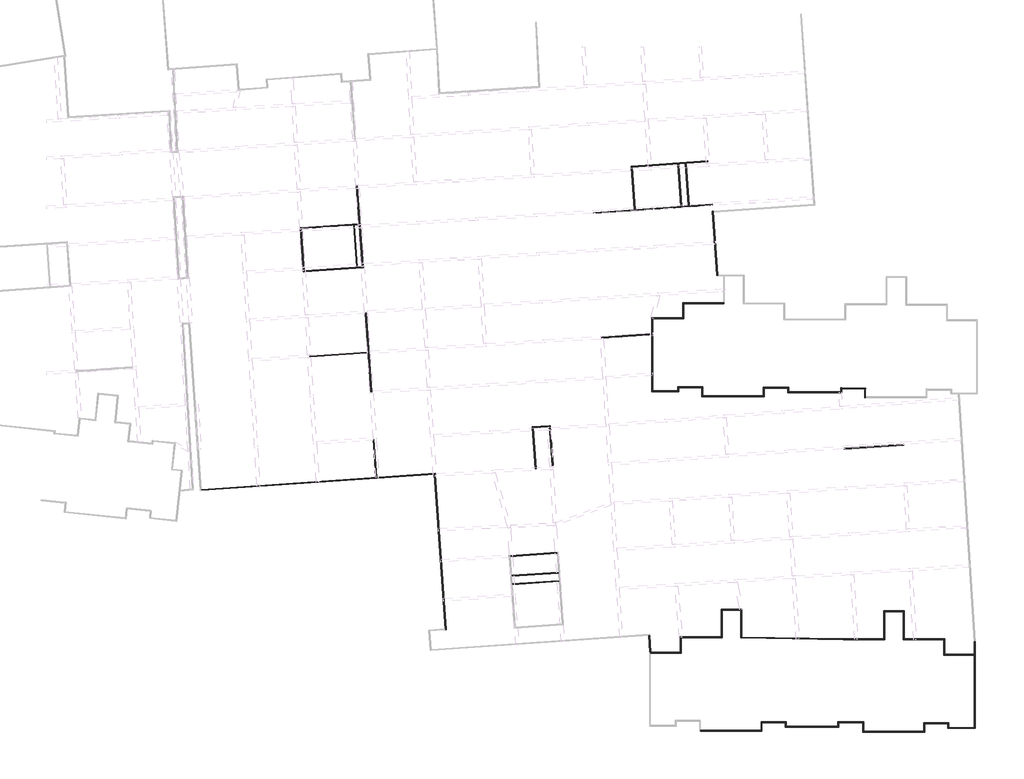
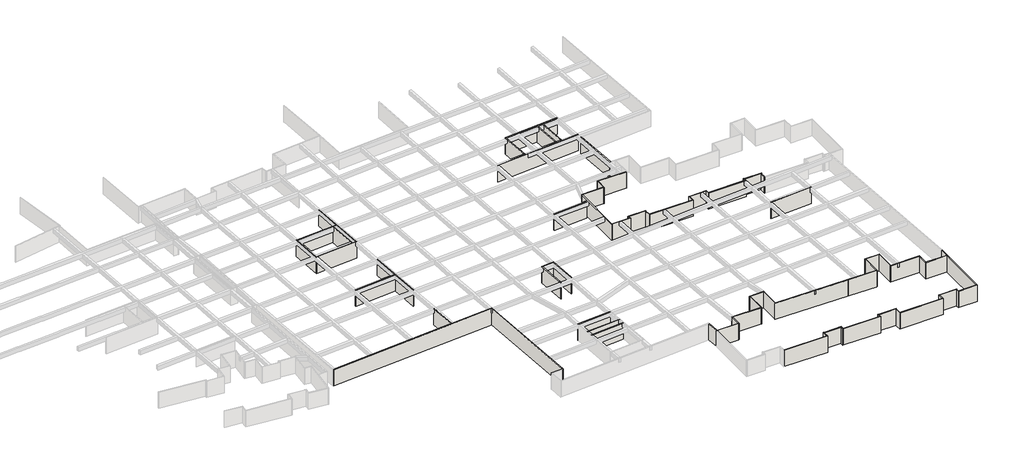
# One storey, part 5 of 14: 69 walls.
"""IFC4 building model written with IfcOpenShell, lengths in millimetres."""

from ifc_helpers import new_model, si_unit, origin, origin_with_axes, place, context, project, spatial, polyline, outline, extrude, faceted_brep, element, save

model = new_model("IFC4")

# Units and contexts
model_context = context("Model", 3, world=origin())
ifc_project = project(units=[si_unit("LENGTHUNIT", "METRE", prefix="MILLI")], contexts=[model_context])

# Site, building, storey
site = spatial("IfcSite", under=ifc_project)
building = spatial("IfcBuilding", under=site)
storey = spatial("IfcBuildingStorey", under=building, Name="户型图", Elevation=0.0)

# Walls
placement = place(None, origin())
element("IfcWall", 1, ObjectType="所有墙体", at=placement, inside=storey, context=model_context, shape_type="Brep", body=[
    faceted_brep([(-67010.794427, -211582.679776, 0.0), (-58619.9111457, -211582.679776, 0.0), (-58619.9111457, -211582.679776, 3300.0), (-67010.794427, -211582.679776, 3300.0), (-67010.794427, -211462.679776, 0.0), (-67010.794427, -211462.679776, 3300.0), (-58739.9111457, -211462.679776, 3300.0), (-58619.9111457, -211462.679776, 3300.0), (-58619.9111457, -211462.679776, 0.0), (-58739.9111457, -211462.679776, 0.0)], [[[0, 1, 2, 3]], [[4, 5, 6, 7, 8, 9]], [[1, 0, 4, 9, 8]], [[3, 2, 7, 6, 5]], [[0, 3, 5, 4]], [[2, 1, 8, 7]]]),
])
element("IfcWall", 2, ObjectType="所有墙体", at=placement, inside=storey, context=model_context, shape_type="Brep", body=[
    faceted_brep([(-58619.9111457, -211462.679776, 0.0), (-58619.9111457, -210441.7795098, 0.0), (-58619.9111457, -210321.7795098, 0.0), (-58619.9111457, -210321.7795098, 3300.0), (-58619.9111457, -210441.7795098, 3300.0), (-58619.9111457, -211462.679776, 3300.0), (-58739.9111457, -211462.679776, 0.0), (-58739.9111457, -211462.679776, 3300.0), (-58739.9111457, -210321.7795098, 3300.0), (-58739.9111457, -210321.7795098, 0.0)], [[[0, 1, 2, 3, 4, 5]], [[6, 7, 8, 9]], [[2, 1, 0, 6, 9]], [[5, 4, 3, 8, 7]], [[0, 5, 7, 6]], [[3, 2, 9, 8]]]),
])
element("IfcWall", 3, ObjectType="所有墙体", at=placement, inside=storey, context=model_context, shape_type="Brep", body=[
    faceted_brep([(-58619.9111457, -210441.7795098, 0.0), (-55431.7894255, -210441.7795098, 0.0), (-55311.7894255, -210441.7795098, 0.0), (-55311.7894255, -210441.7795098, 3300.0), (-55431.7894255, -210441.7795098, 3300.0), (-58619.9111457, -210441.7795098, 3300.0), (-58619.9111457, -210321.7795098, 0.0), (-58619.9111457, -210321.7795098, 3300.0), (-55311.7894255, -210321.7795098, 3300.0), (-55311.7894255, -210321.7795098, 0.0)], [[[0, 1, 2, 3, 4, 5]], [[6, 7, 8, 9]], [[2, 1, 0, 6, 9]], [[5, 4, 3, 8, 7]], [[0, 5, 7, 6]], [[3, 2, 9, 8]]]),
])
element("IfcWall", 4, ObjectType="所有墙体", at=placement, inside=storey, context=model_context, shape_type="Brep", body=[
    faceted_brep([(-55431.7894255, -210441.7795098, 0.0), (-55431.7894255, -211065.1063364, 0.0), (-55431.7894255, -211065.1063364, 3300.0), (-55431.7894255, -210441.7795098, 3300.0), (-55311.7894255, -210441.7795098, 0.0), (-55311.7894255, -210441.7795098, 3300.0), (-55311.7894255, -210945.1063364, 3300.0), (-55311.7894255, -211065.1063364, 3300.0), (-55311.7894255, -211065.1063364, 0.0), (-55311.7894255, -210945.1063364, 0.0)], [[[0, 1, 2, 3]], [[4, 5, 6, 7, 8, 9]], [[1, 0, 4, 9, 8]], [[3, 2, 7, 6, 5]], [[0, 3, 5, 4]], [[2, 1, 8, 7]]]),
])
element("IfcWall", 5, ObjectType="所有墙体", at=placement, inside=storey, context=model_context, shape_type="Brep", body=[
    faceted_brep([(-55311.7894255, -211065.1063364, 0.0), (-48116.0031651, -211065.1063364, 0.0), (-48116.0031651, -211065.1063364, 3300.0), (-55311.7894255, -211065.1063364, 3300.0), (-55311.7894255, -210945.1063364, 0.0), (-55311.7894255, -210945.1063364, 3300.0), (-48236.0031651, -210945.1063364, 3300.0), (-48116.0031651, -210945.1063364, 3300.0), (-48116.0031651, -210945.1063364, 0.0), (-48236.0031651, -210945.1063364, 0.0)], [[[0, 1, 2, 3]], [[4, 5, 6, 7, 8, 9]], [[1, 0, 4, 9, 8]], [[3, 2, 7, 6, 5]], [[0, 3, 5, 4]], [[2, 1, 8, 7]]]),
])
element("IfcWall", 6, ObjectType="所有墙体", at=placement, inside=storey, context=model_context, shape_type="Brep", body=[
    faceted_brep([(-48116.0031651, -210945.1063364, 0.0), (-48116.0031651, -210441.7795098, 0.0), (-48116.0031651, -210321.7795098, 0.0), (-48116.0031651, -210321.7795098, 3300.0), (-48116.0031651, -210441.7795098, 3300.0), (-48116.0031651, -210945.1063364, 3300.0), (-48236.0031651, -210945.1063364, 0.0), (-48236.0031651, -210945.1063364, 3300.0), (-48236.0031651, -210321.7795098, 3300.0), (-48236.0031651, -210321.7795098, 0.0)], [[[0, 1, 2, 3, 4, 5]], [[6, 7, 8, 9]], [[2, 1, 0, 6, 9]], [[5, 4, 3, 8, 7]], [[0, 5, 7, 6]], [[3, 2, 9, 8]]]),
])
element("IfcWall", 7, ObjectType="所有墙体", at=placement, inside=storey, context=model_context, shape_type="Brep", body=[
    faceted_brep([(-48116.0031651, -210441.7795098, 0.0), (-44836.0031651, -210441.7795098, 0.0), (-44716.0031651, -210441.7795098, 0.0), (-44716.0031651, -210441.7795098, 3300.0), (-44836.0031651, -210441.7795098, 3300.0), (-48116.0031651, -210441.7795098, 3300.0), (-48116.0031651, -210321.7795098, 0.0), (-48116.0031651, -210321.7795098, 3300.0), (-44716.0031651, -210321.7795098, 3300.0), (-44716.0031651, -210321.7795098, 0.0)], [[[0, 1, 2, 3, 4, 5]], [[6, 7, 8, 9]], [[2, 1, 0, 6, 9]], [[5, 4, 3, 8, 7]], [[0, 5, 7, 6]], [[3, 2, 9, 8]]]),
])
element("IfcWall", 8, ObjectType="所有墙体", at=placement, inside=storey, context=model_context, shape_type="Brep", body=[
    faceted_brep([(-44836.0031651, -210441.7795098, 0.0), (-44836.0031651, -211739.788444, 0.0), (-44836.0031651, -211739.788444, 3300.0), (-44836.0031651, -210441.7795098, 3300.0), (-44716.0031651, -210441.7795098, 0.0), (-44716.0031651, -210441.7795098, 3300.0), (-44716.0031651, -211619.788444, 3300.0), (-44716.0031651, -211739.788444, 3300.0), (-44716.0031651, -211739.788444, 0.0), (-44716.0031651, -211619.788444, 0.0)], [[[0, 1, 2, 3]], [[4, 5, 6, 7, 8, 9]], [[1, 0, 4, 9, 8]], [[3, 2, 7, 6, 5]], [[0, 3, 5, 4]], [[2, 1, 8, 7]]]),
])
element("IfcWall", 9, ObjectType="所有墙体", at=placement, inside=storey, context=model_context, shape_type="Brep", body=[
    faceted_brep([(-44716.0031651, -211739.788444, 0.0), (-36420.4670689, -211739.788444, 0.0), (-36420.4670689, -211739.788444, 3300.0), (-44716.0031651, -211739.788444, 3300.0), (-44716.0031651, -211619.788444, 0.0), (-44716.0031651, -211619.788444, 3300.0), (-36540.4670689, -211619.788444, 3300.0), (-36420.4670689, -211619.788444, 3300.0), (-36420.4670689, -211619.788444, 0.0), (-36540.4670689, -211619.788444, 0.0)], [[[0, 1, 2, 3]], [[4, 5, 6, 7, 8, 9]], [[1, 0, 4, 9, 8]], [[3, 2, 7, 6, 5]], [[0, 3, 5, 4]], [[2, 1, 8, 7]]]),
])
element("IfcWall", 10, ObjectType="所有墙体", at=placement, inside=storey, context=model_context, shape_type="Brep", body=[
    faceted_brep([(-36420.4670689, -211619.788444, 0.0), (-36420.4670689, -210598.2162779, 0.0), (-36420.4670689, -210478.2162779, 0.0), (-36420.4670689, -210478.2162779, 3300.0), (-36420.4670689, -210598.2162779, 3300.0), (-36420.4670689, -211619.788444, 3300.0), (-36540.4670689, -211619.788444, 0.0), (-36540.4670689, -211619.788444, 3300.0), (-36540.4670689, -210478.2162779, 3300.0), (-36540.4670689, -210478.2162779, 0.0)], [[[0, 1, 2, 3, 4, 5]], [[6, 7, 8, 9]], [[2, 1, 0, 6, 9]], [[5, 4, 3, 8, 7]], [[0, 5, 7, 6]], [[3, 2, 9, 8]]]),
])
element("IfcWall", 11, ObjectType="所有墙体", at=placement, inside=storey, context=model_context, shape_type="Brep", body=[
    faceted_brep([(-36420.4670689, -210598.2162779, 0.0), (-33232.340614, -210598.2162779, 0.0), (-33112.340614, -210598.2162779, 0.0), (-33112.340614, -210598.2162779, 3300.0), (-33232.340614, -210598.2162779, 3300.0), (-36420.4670689, -210598.2162779, 3300.0), (-36420.4670689, -210478.2162779, 0.0), (-36420.4670689, -210478.2162779, 3300.0), (-33112.340614, -210478.2162779, 3300.0), (-33112.340614, -210478.2162779, 0.0)], [[[0, 1, 2, 3, 4, 5]], [[6, 7, 8, 9]], [[2, 1, 0, 6, 9]], [[5, 4, 3, 8, 7]], [[0, 5, 7, 6]], [[3, 2, 9, 8]]]),
])
element("IfcWall", 12, ObjectType="所有墙体", at=placement, inside=storey, context=model_context, shape_type="Brep", body=[
    faceted_brep([(-33232.340614, -210598.2162779, 0.0), (-33232.340614, -211221.5431378, 0.0), (-33232.340614, -211221.5431378, 3300.0), (-33232.340614, -210598.2162779, 3300.0), (-33112.340614, -210598.2162779, 0.0), (-33112.340614, -210598.2162779, 3300.0), (-33112.340614, -211101.5431378, 3300.0), (-33112.340614, -211221.5431378, 3300.0), (-33112.340614, -211221.5431378, 0.0), (-33112.340614, -211101.5431378, 0.0)], [[[0, 1, 2, 3]], [[4, 5, 6, 7, 8, 9]], [[1, 0, 4, 9, 8]], [[3, 2, 7, 6, 5]], [[0, 3, 5, 4]], [[2, 1, 8, 7]]]),
])
element("IfcWall", 13, ObjectType="所有墙体", at=placement, inside=storey, context=model_context, shape_type="Brep", body=[
    faceted_brep([(-33112.340614, -211221.5431378, 0.0), (-29516.643738, -211221.5431378, 0.0), (-29516.643738, -211221.5431378, 3300.0), (-33112.340614, -211221.5431378, 3300.0), (-33112.340614, -211101.5431378, 0.0), (-33112.340614, -211101.5431378, 3300.0), (-29636.643738, -211101.5431378, 3300.0), (-29516.643738, -211101.5431378, 3300.0), (-29516.643738, -211101.5431378, 0.0), (-29636.643738, -211101.5431378, 0.0)], [[[0, 1, 2, 3]], [[4, 5, 6, 7, 8, 9]], [[1, 0, 4, 9, 8]], [[3, 2, 7, 6, 5]], [[0, 3, 5, 4]], [[2, 1, 8, 7]]]),
])
element("IfcWall", 14, ObjectType="所有墙体", at=placement, inside=storey, context=model_context, shape_type="Brep", body=[
    faceted_brep([(-29516.643738, -211101.5431378, 0.0), (-29516.643738, -199359.5961168, 0.0), (-29516.643738, -199359.5961168, 3300.0), (-29516.643738, -211101.5431378, 3300.0), (-29636.643738, -211101.5431378, 0.0), (-29636.643738, -211101.5431378, 3300.0), (-29636.643738, -201221.5431378, 3300.0), (-29636.643738, -201101.5431378, 3300.0), (-29636.643738, -199363.4901589, 3300.0), (-29636.643738, -199363.4901589, 0.0), (-29636.643738, -201101.5431378, 0.0), (-29636.643738, -201221.5431378, 0.0)], [[[0, 1, 2, 3]], [[4, 5, 6, 7, 8, 9, 10, 11]], [[1, 0, 4, 11, 10, 9]], [[3, 2, 8, 7, 6, 5]], [[0, 3, 5, 4]], [[2, 1, 9, 8]]]),
])
element("IfcWall", 15, ObjectType="所有墙体", at=placement, inside=storey, context=model_context, shape_type="Brep", body=[
    faceted_brep([(-29636.643738, -201101.5431378, 0.0), (-33646.2792422, -201101.5431378, 0.0), (-33766.2792422, -201101.5431378, 0.0), (-33766.2792422, -201101.5431378, 3300.0), (-33646.2792422, -201101.5431378, 3300.0), (-29636.643738, -201101.5431378, 3300.0), (-29636.643738, -201221.5431378, 0.0), (-29636.643738, -201221.5431378, 3300.0), (-33766.2792422, -201221.5431378, 3300.0), (-33766.2792422, -201221.5431378, 0.0)], [[[0, 1, 2, 3, 4, 5]], [[6, 7, 8, 9]], [[2, 1, 0, 6, 9]], [[5, 4, 3, 8, 7]], [[0, 5, 7, 6]], [[3, 2, 9, 8]]]),
])
element("IfcWall", 16, ObjectType="所有墙体", at=placement, inside=storey, context=model_context, shape_type="Brep", body=[
    faceted_brep([(-33646.2792422, -201101.5431378, 0.0), (-33646.2792422, -198997.4801078, 0.0), (-33646.2792422, -198997.4801078, 3300.0), (-33646.2792422, -201101.5431378, 3300.0), (-33766.2792422, -201101.5431378, 0.0), (-33766.2792422, -201101.5431378, 3300.0), (-33766.2792422, -199117.4801078, 3300.0), (-33766.2792422, -198997.4801078, 3300.0), (-33766.2792422, -198997.4801078, 0.0), (-33766.2792422, -199117.4801078, 0.0)], [[[0, 1, 2, 3]], [[4, 5, 6, 7, 8, 9]], [[1, 0, 4, 9, 8]], [[3, 2, 7, 6, 5]], [[0, 3, 5, 4]], [[2, 1, 8, 7]]]),
])
element("IfcWall", 17, ObjectType="所有墙体", at=placement, inside=storey, context=model_context, shape_type="Brep", body=[
    faceted_brep([(-33766.2792422, -198997.4801078, 0.0), (-39181.5899679, -198997.4801078, 0.0), (-39301.5899679, -198997.4801078, 0.0), (-39301.5899679, -198997.4801078, 3300.0), (-39181.5899679, -198997.4801078, 3300.0), (-33766.2792422, -198997.4801078, 3300.0), (-33766.2792422, -199117.4801078, 0.0), (-33766.2792422, -199117.4801078, 3300.0), (-39301.5899679, -199117.4801078, 3300.0), (-39301.5899679, -199117.4801078, 0.0)], [[[0, 1, 2, 3, 4, 5]], [[6, 7, 8, 9]], [[2, 1, 0, 6, 9]], [[5, 4, 3, 8, 7]], [[0, 5, 7, 6]], [[3, 2, 9, 8]]]),
])
element("IfcWall", 18, ObjectType="所有墙体", at=placement, inside=storey, context=model_context, shape_type="Brep", body=[
    faceted_brep([(-39181.5899679, -198997.4801078, 0.0), (-39181.5899679, -195158.3790997, 0.0), (-39181.5899679, -195158.3790997, 3300.0), (-39181.5899679, -198997.4801078, 3300.0), (-39301.5899679, -198997.4801078, 0.0), (-39301.5899679, -198997.4801078, 3300.0), (-39301.5899679, -195278.3790997, 3300.0), (-39301.5899679, -195158.3790997, 3300.0), (-39301.5899679, -195158.3790997, 0.0), (-39301.5899679, -195278.3790997, 0.0)], [[[0, 1, 2, 3]], [[4, 5, 6, 7, 8, 9]], [[1, 0, 4, 9, 8]], [[3, 2, 7, 6, 5]], [[0, 3, 5, 4]], [[2, 1, 8, 7]]]),
])
element("IfcWall", 19, ObjectType="所有墙体", at=placement, inside=storey, context=model_context, shape_type="Brep", body=[
    faceted_brep([(-39301.5899679, -195158.3790997, 0.0), (-41974.6033306, -195158.3790997, 0.0), (-41974.6033306, -195158.3790997, 3300.0), (-39301.5899679, -195158.3790997, 3300.0), (-39301.5899679, -195278.3790997, 0.0), (-39301.5899679, -195278.3790997, 3300.0), (-41854.6033306, -195278.3790997, 3300.0), (-41974.6033306, -195278.3790997, 3300.0), (-41974.6033306, -195278.3790997, 0.0), (-41854.6033306, -195278.3790997, 0.0)], [[[0, 1, 2, 3]], [[4, 5, 6, 7, 8, 9]], [[1, 0, 4, 9, 8]], [[3, 2, 7, 6, 5]], [[0, 3, 5, 4]], [[2, 1, 8, 7]]]),
])
element("IfcWall", 20, ObjectType="所有墙体", at=placement, inside=storey, context=model_context, shape_type="Brep", body=[
    faceted_brep([(-41974.6033306, -195278.3790997, 0.0), (-41974.6033306, -198997.4801078, 0.0), (-41974.6033306, -199117.4801078, 0.0), (-41974.6033306, -199117.4801078, 3300.0), (-41974.6033306, -198997.4801078, 3300.0), (-41974.6033306, -195278.3790997, 3300.0), (-41854.6033306, -195278.3790997, 0.0), (-41854.6033306, -195278.3790997, 3300.0), (-41854.6033306, -199117.4801078, 3300.0), (-41854.6033306, -199117.4801078, 0.0)], [[[0, 1, 2, 3, 4, 5]], [[6, 7, 8, 9]], [[2, 1, 0, 6, 9]], [[5, 4, 3, 8, 7]], [[0, 5, 7, 6]], [[3, 2, 9, 8]]]),
])
element("IfcWall", 21, ObjectType="所有墙体", at=placement, inside=storey, context=model_context, shape_type="SweptSolid", body=[
    extrude(outline(polyline([(-47491.2711945, -198997.4801078), (-41974.6033306, -198997.4801078), (-41974.6033306, -199117.4801078), (-47492.3184187, -199117.4801078), (-47491.2711945, -198997.4801078)])), origin_with_axes(), (0.0, 0.0, 1.0), 3300.0),
])
element("IfcWall", 22, ObjectType="所有墙体", at=placement, inside=storey, context=model_context, shape_type="Brep", body=[
    faceted_brep([(-47491.2711945, -198997.4801078, 0.0), (-61380.425437, -198755.0440187, 0.0), (-61500.425437, -198752.9494109, 0.0), (-61500.425437, -198752.9494109, 3300.0), (-61380.425437, -198755.0440187, 3300.0), (-47491.2711945, -198997.4801078, 3300.0), (-47492.3184187, -199117.4801078, 0.0), (-47492.3184187, -199117.4801078, 3300.0), (-61500.425437, -198872.9676903, 3300.0), (-61500.425437, -198872.9676903, 0.0)], [[[0, 1, 2, 3, 4, 5]], [[6, 7, 8, 9]], [[2, 1, 0, 6, 9]], [[5, 4, 3, 8, 7]], [[0, 5, 7, 6]], [[3, 2, 9, 8]]]),
])
element("IfcWall", 23, ObjectType="所有墙体", at=placement, inside=storey, context=model_context, shape_type="Brep", body=[
    faceted_brep([(-61380.425437, -198755.0440187, 0.0), (-61380.425437, -194954.0058545, 0.0), (-61380.425437, -194954.0058545, 3300.0), (-61380.425437, -198755.0440187, 3300.0), (-61500.425437, -198752.9494109, 0.0), (-61500.425437, -198752.9494109, 3300.0), (-61500.425437, -195074.0058545, 3300.0), (-61500.425437, -194954.0058545, 3300.0), (-61500.425437, -194954.0058545, 0.0), (-61500.425437, -195074.0058545, 0.0)], [[[0, 1, 2, 3]], [[4, 5, 6, 7, 8, 9]], [[1, 0, 4, 9, 8]], [[3, 2, 7, 6, 5]], [[0, 3, 5, 4]], [[2, 1, 8, 7]]]),
])
element("IfcWall", 24, ObjectType="所有墙体", at=placement, inside=storey, context=model_context, shape_type="Brep", body=[
    faceted_brep([(-61500.425437, -194954.0058545, 0.0), (-64173.7143397, -194954.0058545, 0.0), (-64173.7143397, -194954.0058545, 3300.0), (-61500.425437, -194954.0058545, 3300.0), (-61500.425437, -195074.0058545, 0.0), (-61500.425437, -195074.0058545, 3300.0), (-64053.7143397, -195074.0058545, 3300.0), (-64173.7143397, -195074.0058545, 3300.0), (-64173.7143397, -195074.0058545, 0.0), (-64053.7143397, -195074.0058545, 0.0)], [[[0, 1, 2, 3]], [[4, 5, 6, 7, 8, 9]], [[1, 0, 4, 9, 8]], [[3, 2, 7, 6, 5]], [[0, 3, 5, 4]], [[2, 1, 8, 7]]]),
])
element("IfcWall", 25, ObjectType="所有墙体", at=placement, inside=storey, context=model_context, shape_type="Brep", body=[
    faceted_brep([(-64173.7143397, -195074.0058545, 0.0), (-64173.7143397, -198707.3434231, 0.0), (-64173.7143397, -198827.3434231, 0.0), (-64173.7143397, -198827.3434231, 3300.0), (-64173.7143397, -198707.3434231, 3300.0), (-64173.7143397, -195074.0058545, 3300.0), (-64053.7143397, -195074.0058545, 0.0), (-64053.7143397, -195074.0058545, 3300.0), (-64053.7143397, -198827.3434231, 3300.0), (-64053.7143397, -198827.3434231, 0.0)], [[[0, 1, 2, 3, 4, 5]], [[6, 7, 8, 9]], [[2, 1, 0, 6, 9]], [[5, 4, 3, 8, 7]], [[0, 5, 7, 6]], [[3, 2, 9, 8]]]),
])
element("IfcWall", 26, ObjectType="所有墙体", at=placement, inside=storey, context=model_context, shape_type="Brep", body=[
    faceted_brep([(-64173.7143397, -198707.3434231, 0.0), (-69750.3014513, -198707.3434231, 0.0), (-69750.3014513, -198707.3434231, 3300.0), (-64173.7143397, -198707.3434231, 3300.0), (-64173.7143397, -198827.3434231, 0.0), (-64173.7143397, -198827.3434231, 3300.0), (-69630.3014513, -198827.3434231, 3300.0), (-69750.3014513, -198827.3434231, 3300.0), (-69750.3014513, -198827.3434231, 0.0), (-69630.3014513, -198827.3434231, 0.0)], [[[0, 1, 2, 3]], [[4, 5, 6, 7, 8, 9]], [[1, 0, 4, 9, 8]], [[3, 2, 7, 6, 5]], [[0, 3, 5, 4]], [[2, 1, 8, 7]]]),
])
element("IfcWall", 27, ObjectType="所有墙体", at=placement, inside=storey, context=model_context, shape_type="Brep", body=[
    faceted_brep([(-69750.3014513, -198827.3434231, 0.0), (-69750.3014513, -200843.9572436, 0.0), (-69750.3014513, -200963.9572436, 0.0), (-69750.3014513, -200963.9572436, 3300.0), (-69750.3014513, -200843.9572436, 3300.0), (-69750.3014513, -198827.3434231, 3300.0), (-69630.3014513, -198827.3434231, 0.0), (-69630.3014513, -198827.3434231, 3300.0), (-69630.3014513, -200963.9572436, 3300.0), (-69630.3014513, -200963.9572436, 0.0)], [[[0, 1, 2, 3, 4, 5]], [[6, 7, 8, 9]], [[2, 1, 0, 6, 9]], [[5, 4, 3, 8, 7]], [[0, 5, 7, 6]], [[3, 2, 9, 8]]]),
])
element("IfcWall", 28, ObjectType="所有墙体", at=placement, inside=storey, context=model_context, shape_type="Brep", body=[
    faceted_brep([(-69750.3014513, -200843.9572436, 0.0), (-73794.4999662, -200843.9572436, 0.0), (-73845.252881, -200843.9572436, 0.0), (-73845.252881, -200843.9572436, 3300.0), (-73794.4999662, -200843.9572436, 3300.0), (-69750.3014513, -200843.9572436, 3300.0), (-69750.3014513, -200963.9572436, 0.0), (-69750.3014513, -200963.9572436, 3300.0), (-73845.252881, -200963.9572436, 3300.0), (-73845.252881, -200963.9572436, 0.0)], [[[0, 1, 2, 3, 4, 5]], [[6, 7, 8, 9]], [[2, 1, 0, 6, 9]], [[5, 4, 3, 8, 7]], [[3, 2, 9, 8]], [[0, 5, 7, 6]]]),
])
element("IfcWall", 29, ObjectType="所有墙体", at=placement, inside=storey, context=model_context, shape_type="Brep", body=[
    faceted_brep([(-63852.357784, -153118.7611434, 0.0), (-69429.0689186, -153118.7611434, 0.0), (-69429.0689186, -153118.7611434, 3300.0), (-63852.357784, -153118.7611434, 3300.0), (-63852.357784, -153238.7611434, 0.0), (-63852.357784, -153238.7611434, 3300.0), (-69309.0689186, -153238.7611434, 3300.0), (-69429.0689186, -153238.7611434, 3300.0), (-69429.0689186, -153238.7611434, 0.0), (-69309.0689186, -153238.7611434, 0.0)], [[[0, 1, 2, 3]], [[4, 5, 6, 7, 8, 9]], [[1, 0, 4, 9, 8]], [[3, 2, 7, 6, 5]], [[0, 3, 5, 4]], [[2, 1, 8, 7]]]),
])
element("IfcWall", 30, ObjectType="所有墙体", at=placement, inside=storey, context=model_context, shape_type="Brep", body=[
    faceted_brep([(-69429.0689186, -153238.7611434, 0.0), (-69429.0689186, -155179.8125449, 0.0), (-69429.0689186, -155299.8125449, 0.0), (-69429.0689186, -155299.8125449, 3300.0), (-69429.0689186, -155179.8125449, 3300.0), (-69429.0689186, -153238.7611434, 3300.0), (-69309.0689186, -153238.7611434, 0.0), (-69309.0689186, -153238.7611434, 3300.0), (-69309.0689186, -155299.8125449, 3300.0), (-69309.0689186, -155299.8125449, 0.0)], [[[0, 1, 2, 3, 4, 5]], [[6, 7, 8, 9]], [[2, 1, 0, 6, 9]], [[5, 4, 3, 8, 7]], [[0, 5, 7, 6]], [[3, 2, 9, 8]]]),
])
element("IfcWall", 31, ObjectType="所有墙体", at=placement, inside=storey, context=model_context, shape_type="Brep", body=[
    faceted_brep([(-69429.0689186, -155179.8125449, 0.0), (-73643.5852972, -155179.8125449, 0.0), (-73643.5852972, -155179.8125449, 3300.0), (-69429.0689186, -155179.8125449, 3300.0), (-69429.0689186, -155299.8125449, 0.0), (-69429.0689186, -155299.8125449, 3300.0), (-73523.5852972, -155299.8125449, 3300.0), (-73643.5852972, -155299.8125449, 3300.0), (-73643.5852972, -155299.8125449, 0.0), (-73523.5852972, -155299.8125449, 0.0)], [[[0, 1, 2, 3]], [[4, 5, 6, 7, 8, 9]], [[1, 0, 4, 9, 8]], [[3, 2, 7, 6, 5]], [[0, 3, 5, 4]], [[2, 1, 8, 7]]]),
])
element("IfcWall", 32, ObjectType="所有墙体", at=placement, inside=storey, context=model_context, shape_type="Brep", body=[
    faceted_brep([(-73643.5852972, -155299.8125449, 0.0), (-73643.5852972, -165270.5834458, 0.0), (-73643.5852972, -165270.5834458, 3300.0), (-73643.5852972, -155299.8125449, 3300.0), (-73523.5852972, -155299.8125449, 0.0), (-73523.5852972, -155299.8125449, 3300.0), (-73523.5852972, -165150.5834458, 3300.0), (-73523.5852972, -165270.5834458, 3300.0), (-73523.5852972, -165270.5834458, 0.0), (-73523.5852972, -165150.5834458, 0.0)], [[[0, 1, 2, 3]], [[4, 5, 6, 7, 8, 9]], [[1, 0, 4, 9, 8]], [[3, 2, 7, 6, 5]], [[0, 3, 5, 4]], [[2, 1, 8, 7]]]),
])
element("IfcWall", 33, ObjectType="所有墙体", at=placement, inside=storey, context=model_context, shape_type="Brep", body=[
    faceted_brep([(-73523.5852972, -165270.5834458, 0.0), (-69993.2264591, -165270.5834458, 0.0), (-69993.2264591, -165270.5834458, 3300.0), (-73523.5852972, -165270.5834458, 3300.0), (-73523.5852972, -165150.5834458, 0.0), (-73523.5852972, -165150.5834458, 3300.0), (-70113.2264591, -165150.5834458, 3300.0), (-69993.2264591, -165150.5834458, 3300.0), (-69993.2264591, -165150.5834458, 0.0), (-70113.2264591, -165150.5834458, 0.0)], [[[0, 1, 2, 3]], [[4, 5, 6, 7, 8, 9]], [[1, 0, 4, 9, 8]], [[3, 2, 7, 6, 5]], [[0, 3, 5, 4]], [[2, 1, 8, 7]]]),
])
element("IfcWall", 34, ObjectType="所有墙体", at=placement, inside=storey, context=model_context, shape_type="Brep", body=[
    faceted_brep([(-69993.2264591, -165150.5834458, 0.0), (-69993.2264591, -164695.2578452, 0.0), (-69993.2264591, -164575.2578452, 0.0), (-69993.2264591, -164575.2578452, 3300.0), (-69993.2264591, -164695.2578452, 3300.0), (-69993.2264591, -165150.5834458, 3300.0), (-70113.2264591, -165150.5834458, 0.0), (-70113.2264591, -165150.5834458, 3300.0), (-70113.2264591, -164575.2578452, 3300.0), (-70113.2264591, -164575.2578452, 0.0)], [[[0, 1, 2, 3, 4, 5]], [[6, 7, 8, 9]], [[2, 1, 0, 6, 9]], [[5, 4, 3, 8, 7]], [[0, 5, 7, 6]], [[3, 2, 9, 8]]]),
])
element("IfcWall", 35, ObjectType="所有墙体", at=placement, inside=storey, context=model_context, shape_type="Brep", body=[
    faceted_brep([(-69993.2264591, -164695.2578452, 0.0), (-66809.1223042, -164695.2578452, 0.0), (-66689.1223042, -164695.2578452, 0.0), (-66689.1223042, -164695.2578452, 3300.0), (-66809.1223042, -164695.2578452, 3300.0), (-69993.2264591, -164695.2578452, 3300.0), (-69993.2264591, -164575.2578452, 0.0), (-69993.2264591, -164575.2578452, 3300.0), (-66689.1223042, -164575.2578452, 3300.0), (-66689.1223042, -164575.2578452, 0.0)], [[[0, 1, 2, 3, 4, 5]], [[6, 7, 8, 9]], [[2, 1, 0, 6, 9]], [[5, 4, 3, 8, 7]], [[0, 5, 7, 6]], [[3, 2, 9, 8]]]),
])
element("IfcWall", 36, ObjectType="所有墙体", at=placement, inside=storey, context=model_context, shape_type="Brep", body=[
    faceted_brep([(-66809.1223042, -164695.2578452, 0.0), (-66809.1223042, -165918.39398, 0.0), (-66809.1223042, -165918.39398, 3300.0), (-66809.1223042, -164695.2578452, 3300.0), (-66689.1223042, -164695.2578452, 0.0), (-66689.1223042, -164695.2578452, 3300.0), (-66689.1223042, -165798.39398, 3300.0), (-66689.1223042, -165918.39398, 3300.0), (-66689.1223042, -165918.39398, 0.0), (-66689.1223042, -165798.39398, 0.0)], [[[0, 1, 2, 3]], [[4, 5, 6, 7, 8, 9]], [[1, 0, 4, 9, 8]], [[3, 2, 7, 6, 5]], [[0, 3, 5, 4]], [[2, 1, 8, 7]]]),
])
element("IfcWall", 37, ObjectType="所有墙体", at=placement, inside=storey, context=model_context, shape_type="Brep", body=[
    faceted_brep([(-66689.1223042, -165918.39398, 0.0), (-58297.4707286, -165918.39398, 0.0), (-58297.4707286, -165918.39398, 3300.0), (-66689.1223042, -165918.39398, 3300.0), (-66689.1223042, -165798.39398, 0.0), (-66689.1223042, -165798.39398, 3300.0), (-58417.4707286, -165798.39398, 3300.0), (-58297.4707286, -165798.39398, 3300.0), (-58297.4707286, -165798.39398, 0.0), (-58417.4707286, -165798.39398, 0.0)], [[[0, 1, 2, 3]], [[4, 5, 6, 7, 8, 9]], [[1, 0, 4, 9, 8]], [[3, 2, 7, 6, 5]], [[0, 3, 5, 4]], [[2, 1, 8, 7]]]),
])
element("IfcWall", 38, ObjectType="所有墙体", at=placement, inside=storey, context=model_context, shape_type="Brep", body=[
    faceted_brep([(-58297.4707286, -165798.39398, 0.0), (-58297.4707286, -164777.0504792, 0.0), (-58297.4707286, -164657.0504792, 0.0), (-58297.4707286, -164657.0504792, 3300.0), (-58297.4707286, -164777.0504792, 3300.0), (-58297.4707286, -165798.39398, 3300.0), (-58417.4707286, -165798.39398, 0.0), (-58417.4707286, -165798.39398, 3300.0), (-58417.4707286, -164657.0504792, 3300.0), (-58417.4707286, -164657.0504792, 0.0)], [[[0, 1, 2, 3, 4, 5]], [[6, 7, 8, 9]], [[2, 1, 0, 6, 9]], [[5, 4, 3, 8, 7]], [[0, 5, 7, 6]], [[3, 2, 9, 8]]]),
])
element("IfcWall", 39, ObjectType="所有墙体", at=placement, inside=storey, context=model_context, shape_type="Brep", body=[
    faceted_brep([(-58297.4707286, -164777.0504792, 0.0), (-55109.4082066, -164777.0504792, 0.0), (-54989.4082066, -164777.0504792, 0.0), (-54989.4082066, -164777.0504792, 3300.0), (-55109.4082066, -164777.0504792, 3300.0), (-58297.4707286, -164777.0504792, 3300.0), (-58297.4707286, -164657.0504792, 0.0), (-58297.4707286, -164657.0504792, 3300.0), (-54989.4082066, -164657.0504792, 3300.0), (-54989.4082066, -164657.0504792, 0.0)], [[[0, 1, 2, 3, 4, 5]], [[6, 7, 8, 9]], [[2, 1, 0, 6, 9]], [[5, 4, 3, 8, 7]], [[0, 5, 7, 6]], [[3, 2, 9, 8]]]),
])
element("IfcWall", 40, ObjectType="所有墙体", at=placement, inside=storey, context=model_context, shape_type="Brep", body=[
    faceted_brep([(-55109.4082066, -164777.0504792, 0.0), (-55109.4082066, -165400.1996242, 0.0), (-55109.4082066, -165400.1996242, 3300.0), (-55109.4082066, -164777.0504792, 3300.0), (-54989.4082066, -164777.0504792, 0.0), (-54989.4082066, -164777.0504792, 3300.0), (-54989.4082066, -165280.1996242, 3300.0), (-54989.4082066, -165400.1996242, 3300.0), (-54989.4082066, -165400.1996242, 0.0), (-54989.4082066, -165280.1996242, 0.0)], [[[0, 1, 2, 3]], [[4, 5, 6, 7, 8, 9]], [[1, 0, 4, 9, 8]], [[3, 2, 7, 6, 5]], [[0, 3, 5, 4]], [[2, 1, 8, 7]]]),
])
element("IfcWall", 41, ObjectType="所有墙体", at=placement, inside=storey, context=model_context, shape_type="Brep", body=[
    faceted_brep([(-54989.4082066, -165400.1996242, 0.0), (-47743.588827, -165400.1996242, 0.0), (-47743.588827, -165400.1996242, 3300.0), (-54989.4082066, -165400.1996242, 3300.0), (-54989.4082066, -165280.1996242, 0.0), (-54989.4082066, -165280.1996242, 3300.0), (-47863.588827, -165280.1996242, 3300.0), (-47743.588827, -165280.1996242, 3300.0), (-47743.588827, -165280.1996242, 0.0), (-47863.588827, -165280.1996242, 0.0)], [[[0, 1, 2, 3]], [[4, 5, 6, 7, 8, 9]], [[1, 0, 4, 9, 8]], [[3, 2, 7, 6, 5]], [[0, 3, 5, 4]], [[2, 1, 8, 7]]]),
])
element("IfcWall", 42, ObjectType="所有墙体", at=placement, inside=storey, context=model_context, shape_type="Brep", body=[
    faceted_brep([(-47743.588827, -165280.1996242, 0.0), (-47743.588827, -164877.0504792, 0.0), (-47743.588827, -164757.0504792, 0.0), (-47743.588827, -164717.0504792, 0.0), (-47743.588827, -164717.0504792, 3300.0), (-47743.588827, -164757.0504792, 3300.0), (-47743.588827, -164877.0504792, 3300.0), (-47743.588827, -165280.1996242, 3300.0), (-47863.588827, -165280.1996242, 0.0), (-47863.588827, -165280.1996242, 3300.0), (-47863.588827, -164717.0504792, 3300.0), (-47863.588827, -164717.0504792, 0.0)], [[[0, 1, 2, 3, 4, 5, 6, 7]], [[8, 9, 10, 11]], [[3, 2, 1, 0, 8, 11]], [[4, 3, 11, 10]], [[7, 6, 5, 4, 10, 9]], [[0, 7, 9, 8]]]),
])
element("IfcWall", 43, ObjectType="所有墙体", at=placement, inside=storey, context=model_context, shape_type="Brep", body=[
    faceted_brep([(-47743.588827, -164877.0504792, 0.0), (-44609.8483382, -164877.0504792, 0.0), (-44489.8483382, -164877.0504792, 0.0), (-44449.8483382, -164877.0504792, 0.0), (-44449.8483382, -164877.0504792, 3300.0), (-44489.8483382, -164877.0504792, 3300.0), (-44609.8483382, -164877.0504792, 3300.0), (-47743.588827, -164877.0504792, 3300.0), (-47743.588827, -164757.0504792, 0.0), (-47743.588827, -164757.0504792, 3300.0), (-44449.8483382, -164757.0504792, 3300.0), (-44449.8483382, -164757.0504792, 0.0)], [[[0, 1, 2, 3, 4, 5, 6, 7]], [[8, 9, 10, 11]], [[3, 2, 1, 0, 8, 11]], [[4, 3, 11, 10]], [[7, 6, 5, 4, 10, 9]], [[0, 7, 9, 8]]]),
])
element("IfcWall", 44, ObjectType="所有墙体", at=placement, inside=storey, context=model_context, shape_type="Brep", body=[
    faceted_brep([(-44609.8483382, -164877.0504792, 0.0), (-44609.8483382, -166077.0504792, 0.0), (-44609.8483382, -166077.0504792, 3300.0), (-44609.8483382, -164877.0504792, 3300.0), (-44489.8483382, -164877.0504792, 0.0), (-44489.8483382, -164877.0504792, 3300.0), (-44489.8483382, -165957.0504792, 3300.0), (-44489.8483382, -166077.0504792, 3300.0), (-44489.8483382, -166077.0504792, 0.0), (-44489.8483382, -165957.0504792, 0.0)], [[[0, 1, 2, 3]], [[4, 5, 6, 7, 8, 9]], [[1, 0, 4, 9, 8]], [[3, 2, 7, 6, 5]], [[0, 3, 5, 4]], [[2, 1, 8, 7]]]),
])
element("IfcWall", 45, ObjectType="所有墙体", at=placement, inside=storey, context=model_context, shape_type="Brep", body=[
    faceted_brep([(-135152.7273653, -178738.1882395, 0.0), (-103350.385443, -176514.3518565, 0.0), (-103230.677757, -176505.9810797, 0.0), (-103230.677757, -176505.9810797, 3300.0), (-103350.385443, -176514.3518565, 3300.0), (-135152.7273653, -178738.1882395, 3300.0), (-135161.0981421, -178618.4805535, 0.0), (-135161.0981421, -178618.4805535, 3300.0), (-111353.8592747, -176953.7162383, 3300.0), (-111234.1515887, -176945.3454614, 3300.0), (-103239.0485338, -176386.2733937, 3300.0), (-103239.0485338, -176386.2733937, 0.0), (-111234.1515887, -176945.3454614, 0.0), (-111353.8592747, -176953.7162383, 0.0)], [[[0, 1, 2, 3, 4, 5]], [[6, 7, 8, 9, 10, 11, 12, 13]], [[2, 1, 0, 6, 13, 12, 11]], [[5, 4, 3, 10, 9, 8, 7]], [[0, 5, 7, 6]], [[3, 2, 11, 10]]]),
])
element("IfcWall", 46, ObjectType="所有墙体", at=placement, inside=storey, context=model_context, shape_type="Brep", body=[
    faceted_brep([(-103350.385443, -176514.3518565, 0.0), (-101872.9433291, -197642.758441, 0.0), (-101864.5725522, -197762.4661271, 0.0), (-101864.5725522, -197762.4661271, 3300.0), (-101872.9433291, -197642.758441, 3300.0), (-103350.385443, -176514.3518565, 3300.0), (-103230.677757, -176505.9810797, 0.0), (-103230.677757, -176505.9810797, 3300.0), (-101744.8648662, -197754.0953502, 3300.0), (-101744.8648662, -197754.0953502, 0.0)], [[[0, 1, 2, 3, 4, 5]], [[6, 7, 8, 9]], [[2, 1, 0, 6, 9]], [[5, 4, 3, 8, 7]], [[0, 5, 7, 6]], [[3, 2, 9, 8]]]),
])
element("IfcWall", 47, ObjectType="所有墙体", at=placement, inside=storey, context=model_context, shape_type="Brep", body=[
    faceted_brep([(-74079.2932006, -198491.4946901, 0.0), (-73914.792994, -200843.9572436, 0.0), (-73914.792994, -200843.9572436, 3300.0), (-74079.2932006, -198491.4946901, 3300.0), (-73959.5855146, -198483.1239133, 0.0), (-73959.5855146, -198483.1239133, 3300.0), (-73794.4999662, -200843.9572436, 3300.0), (-73794.4999662, -200843.9572436, 0.0), (-73845.252881, -200843.9572436, 0.0), (-73845.252881, -200843.9572436, 3300.0)], [[[0, 1, 2, 3]], [[4, 5, 6, 7]], [[1, 0, 4, 7, 8]], [[3, 2, 9, 6, 5]], [[2, 1, 8, 7, 6, 9]], [[0, 3, 5, 4]]]),
])
element("IfcWall", 48, ObjectType="所有墙体", at=placement, inside=storey, context=model_context, shape_type="Brep", body=[
    faceted_brep([(-64662.1102247, -149318.6682209, 0.0), (-65261.5124919, -140746.8164451, 0.0), (-65269.8832687, -140627.1087591, 0.0), (-65269.8832687, -140627.1087591, 3300.0), (-65261.5124919, -140746.8164451, 3300.0), (-64662.1102247, -149318.6682209, 3300.0), (-64782.4032525, -149318.6682209, 0.0), (-64782.4032525, -149318.6682209, 3300.0), (-65389.5909547, -140635.4795359, 3300.0), (-65389.5909547, -140635.4795359, 0.0)], [[[0, 1, 2, 3, 4, 5]], [[6, 7, 8, 9]], [[2, 1, 0, 6, 9]], [[5, 4, 3, 8, 7]], [[0, 5, 7, 6]], [[3, 2, 9, 8]]]),
])
element("IfcWall", 49, ObjectType="所有墙体", at=placement, inside=storey, context=model_context, shape_type="Brep", body=[
    faceted_brep([(-121668.4387303, -142878.4869069, 0.0), (-121248.5047584, -148883.8224895, 0.0), (-121248.5047584, -148883.8224895, 3300.0), (-121668.4387303, -142878.4869069, 3300.0), (-121548.7310443, -142870.1161301, 0.0), (-121548.7310443, -142870.1161301, 3300.0), (-121540.3602674, -142989.8238161, 3300.0), (-121137.1678492, -148755.7440266, 3300.0), (-121128.7970723, -148875.4517126, 3300.0), (-121128.7970723, -148875.4517126, 0.0), (-121137.1678492, -148755.7440266, 0.0), (-121540.3602674, -142989.8238161, 0.0)], [[[0, 1, 2, 3]], [[4, 5, 6, 7, 8, 9, 10, 11]], [[1, 0, 4, 11, 10, 9]], [[3, 2, 8, 7, 6, 5]], [[2, 1, 9, 8]], [[0, 3, 5, 4]]]),
])
element("IfcWall", 50, ObjectType="所有墙体", at=placement, inside=storey, context=model_context, shape_type="Brep", body=[
    faceted_brep([(-121128.7970723, -148875.4517126, 0.0), (-113075.9754238, -148312.3435676, 0.0), (-113075.9754238, -148312.3435676, 3300.0), (-121128.7970723, -148875.4517126, 3300.0), (-121137.1678492, -148755.7440266, 0.0), (-121137.1678492, -148755.7440266, 3300.0), (-113962.2025649, -148254.0215785, 3300.0), (-113842.4948789, -148245.6508016, 3300.0), (-113204.0538867, -148201.0066584, 3300.0), (-113084.3462007, -148192.6358816, 3300.0), (-113084.3462007, -148192.6358816, 0.0), (-113204.0538867, -148201.0066584, 0.0), (-113842.4948789, -148245.6508016, 0.0), (-113962.2025649, -148254.0215785, 0.0)], [[[0, 1, 2, 3]], [[4, 5, 6, 7, 8, 9, 10, 11, 12, 13]], [[1, 0, 4, 13, 12, 11, 10]], [[3, 2, 9, 8, 7, 6, 5]], [[0, 3, 5, 4]], [[2, 1, 10, 9]]]),
])
element("IfcWall", 51, ObjectType="所有墙体", at=placement, inside=storey, context=model_context, shape_type="Brep", body=[
    faceted_brep([(-113084.3462007, -148192.6358816, 0.0), (-113857.8498314, -137131.0186105, 0.0), (-113857.8498314, -137131.0186105, 3300.0), (-113084.3462007, -148192.6358816, 3300.0), (-113204.0538867, -148201.0066584, 0.0), (-113204.0538867, -148201.0066584, 3300.0), (-113607.2463049, -142435.0864479, 3300.0), (-113615.6170818, -142315.3787619, 3300.0), (-113977.5575174, -137139.3893874, 3300.0), (-113977.5575174, -137139.3893874, 0.0), (-113615.6170818, -142315.3787619, 0.0), (-113607.2463049, -142435.0864479, 0.0)], [[[0, 1, 2, 3]], [[4, 5, 6, 7, 8, 9, 10, 11]], [[1, 0, 4, 11, 10, 9]], [[2, 1, 9, 8]], [[3, 2, 8, 7, 6, 5]], [[0, 3, 5, 4]]]),
])
element("IfcWall", 52, ObjectType="所有墙体", at=placement, inside=storey, context=model_context, shape_type="Brep", body=[
    faceted_brep([(-121540.3602674, -142989.8238161, 0.0), (-114365.3949831, -142488.101368, 0.0), (-114245.6872971, -142479.7305911, 0.0), (-113607.2463049, -142435.0864479, 0.0), (-113607.2463049, -142435.0864479, 3300.0), (-114245.6872971, -142479.7305911, 3300.0), (-114365.3949831, -142488.101368, 3300.0), (-121540.3602674, -142989.8238161, 3300.0), (-121548.7310443, -142870.1161301, 0.0), (-121548.7310443, -142870.1161301, 3300.0), (-113615.6170818, -142315.3787619, 3300.0), (-113615.6170818, -142315.3787619, 0.0)], [[[0, 1, 2, 3, 4, 5, 6, 7]], [[8, 9, 10, 11]], [[3, 2, 1, 0, 8, 11]], [[7, 6, 5, 4, 10, 9]], [[0, 7, 9, 8]], [[4, 3, 11, 10]]]),
])
element("IfcWall", 53, ObjectType="所有墙体", at=placement, inside=storey, context=model_context, shape_type="SweptSolid", body=[
    extrude(outline(polyline([(-113962.2025649, -148254.0215785), (-114365.3949831, -142488.101368), (-114245.6872971, -142479.7305911), (-113842.4948789, -148245.6508016), (-113962.2025649, -148254.0215785)])), origin_with_axes(), (0.0, 0.0, 1.0), 3300.0),
])
element("IfcWall", 54, ObjectType="所有墙体", at=placement, inside=storey, context=model_context, shape_type="Brep", body=[
    faceted_brep([(-81559.9119656, -140918.9765038, 0.0), (-65388.6937619, -139788.1747695, 0.0), (-65388.6937619, -139788.1747695, 3300.0), (-81559.9119656, -140918.9765038, 3300.0), (-81568.2827424, -140799.2688177, 0.0), (-81568.2827424, -140799.2688177, 3300.0), (-76044.2244366, -140412.9890314, 3300.0), (-75924.5167506, -140404.6182546, 3300.0), (-69709.5947346, -139970.0285715, 3300.0), (-69589.8870486, -139961.6577947, 3300.0), (-68652.1768414, -139896.0867093, 3300.0), (-68532.4691553, -139887.7159325, 3300.0), (-65397.0645388, -139668.4670835, 3300.0), (-65397.0645388, -139668.4670835, 0.0), (-68532.4691553, -139887.7159325, 0.0), (-68652.1768414, -139896.0867093, 0.0), (-69589.8870486, -139961.6577947, 0.0), (-69709.5947346, -139970.0285715, 0.0), (-75924.5167506, -140404.6182546, 0.0), (-76044.2244366, -140412.9890314, 0.0)], [[[0, 1, 2, 3]], [[4, 5, 6, 7, 8, 9, 10, 11, 12, 13, 14, 15, 16, 17, 18, 19]], [[1, 0, 4, 19, 18, 17, 16, 15, 14, 13]], [[2, 1, 13, 12]], [[3, 2, 12, 11, 10, 9, 8, 7, 6, 5]], [[0, 3, 5, 4]]]),
])
element("IfcWall", 55, ObjectType="所有墙体", at=placement, inside=storey, context=model_context, shape_type="Brep", body=[
    faceted_brep([(-76452.2271919, -134578.2777958, 0.0), (-76332.5195059, -134569.9070189, 0.0), (-70117.59749, -134135.3173358, 0.0), (-69997.8898039, -134126.946559, 0.0), (-69060.1795967, -134061.3754737, 0.0), (-68940.4719107, -134053.0046968, 0.0), (-66017.7072262, -133848.6250804, 0.0), (-66017.7072262, -133848.6250804, 3300.0), (-68940.4719107, -134053.0046968, 3300.0), (-69060.1795967, -134061.3754737, 3300.0), (-69997.8898039, -134126.946559, 3300.0), (-70117.59749, -134135.3173358, 3300.0), (-76332.5195059, -134569.9070189, 3300.0), (-76452.2271919, -134578.2777958, 3300.0), (-76460.5979688, -134458.5701097, 0.0), (-76460.5979688, -134458.5701097, 3300.0), (-66026.0780031, -133728.9173944, 3300.0), (-66026.0780031, -133728.9173944, 0.0)], [[[0, 1, 2, 3, 4, 5, 6, 7, 8, 9, 10, 11, 12, 13]], [[14, 15, 16, 17]], [[6, 5, 4, 3, 2, 1, 0, 14, 17]], [[7, 6, 17, 16]], [[13, 12, 11, 10, 9, 8, 7, 16, 15]], [[0, 13, 15, 14]]]),
])
element("IfcWall", 56, ObjectType="所有墙体", at=placement, inside=storey, context=model_context, shape_type="SweptSolid", body=[
    extrude(outline(polyline([(-76044.2244366, -140412.9890314), (-76452.2271919, -134578.2777958), (-76332.5195059, -134569.9070189), (-75924.5167506, -140404.6182546), (-76044.2244366, -140412.9890314)])), origin_with_axes(), (0.0, 0.0, 1.0), 3300.0),
])
element("IfcWall", 57, ObjectType="所有墙体", at=placement, inside=storey, context=model_context, shape_type="SweptSolid", body=[
    extrude(outline(polyline([(-69709.5947346, -139970.0285715), (-70117.59749, -134135.3173358), (-69997.8898039, -134126.946559), (-69589.8870486, -139961.6577947), (-69709.5947346, -139970.0285715)])), origin_with_axes(), (0.0, 0.0, 1.0), 3300.0),
])
element("IfcWall", 58, ObjectType="所有墙体", at=placement, inside=storey, context=model_context, shape_type="SweptSolid", body=[
    extrude(outline(polyline([(-68940.4719107, -134053.0046968), (-68532.4691553, -139887.7159325), (-68652.1768414, -139896.0867093), (-69060.1795967, -134061.3754737), (-68940.4719107, -134053.0046968)])), origin_with_axes(), (0.0, 0.0, 1.0), 3300.0),
])
element("IfcWall", 59, ObjectType="所有墙体", at=placement, inside=storey, context=model_context, shape_type="Brep", body=[
    faceted_brep([(-87138.6732373, -175320.571992, 0.0), (-87519.5435839, -169873.8722775, 0.0), (-87519.5435839, -169873.8722775, 3300.0), (-87138.6732373, -175320.571992, 3300.0), (-87258.3809233, -175328.9427688, 0.0), (-87258.3809233, -175328.9427688, 3300.0), (-87630.8804931, -170001.9507404, 3300.0), (-87639.25127, -169882.2430544, 3300.0), (-87639.25127, -169882.2430544, 0.0), (-87630.8804931, -170001.9507404, 0.0)], [[[0, 1, 2, 3]], [[4, 5, 6, 7, 8, 9]], [[1, 0, 4, 9, 8]], [[3, 2, 7, 6, 5]], [[0, 3, 5, 4]], [[2, 1, 8, 7]]]),
])
element("IfcWall", 60, ObjectType="所有墙体", at=placement, inside=storey, context=model_context, shape_type="Brep", body=[
    faceted_brep([(-87639.25127, -169882.2430544, 0.0), (-89953.6011786, -170044.0781652, 0.0), (-89953.6011786, -170044.0781652, 3300.0), (-87639.25127, -169882.2430544, 3300.0), (-87630.8804931, -170001.9507404, 0.0), (-87630.8804931, -170001.9507404, 3300.0), (-89825.5227157, -170155.4150744, 3300.0), (-89945.2304017, -170163.7858513, 3300.0), (-89945.2304017, -170163.7858513, 0.0), (-89825.5227157, -170155.4150744, 0.0)], [[[0, 1, 2, 3]], [[4, 5, 6, 7, 8, 9]], [[1, 0, 4, 9, 8]], [[3, 2, 7, 6, 5]], [[0, 3, 5, 4]], [[2, 1, 8, 7]]]),
])
element("IfcWall", 61, ObjectType="所有墙体", at=placement, inside=storey, context=model_context, shape_type="SweptSolid", body=[
    extrude(outline(polyline([(-89551.5002895, -175794.3887813), (-89945.2304017, -170163.7858513), (-89825.5227157, -170155.4150744), (-89431.7926035, -175786.0180045), (-89551.5002895, -175794.3887813)])), origin_with_axes(), (0.0, 0.0, 1.0), 3300.0),
])
element("IfcWall", 62, ObjectType="所有墙体", at=placement, inside=storey, context=model_context, shape_type="SweptSolid", body=[
    extrude(outline(polyline([(-80494.2281541, -157801.5421785), (-74010.0618274, -157348.1250992), (-74001.6910505, -157467.8327852), (-80485.8573772, -157921.2498646), (-80494.2281541, -157801.5421785)])), origin_with_axes(), (0.0, 0.0, 1.0), 3300.0),
])
element("IfcWall", 63, ObjectType="所有墙体", at=placement, inside=storey, context=model_context, shape_type="Brep", body=[
    faceted_brep([(-112763.1929726, -154505.6114561, 0.0), (-112390.6934028, -159832.6034845, 0.0), (-112382.322626, -159952.3111705, 0.0), (-112009.8230562, -165279.3031989, 0.0), (-112009.8230562, -165279.3031989, 3300.0), (-112382.322626, -159952.3111705, 3300.0), (-112390.6934028, -159832.6034845, 3300.0), (-112763.1929726, -154505.6114561, 3300.0), (-112643.4852866, -154497.2406792, 0.0), (-112643.4852866, -154497.2406792, 3300.0), (-111890.1153702, -165270.932422, 3300.0), (-111890.1153702, -165270.932422, 0.0)], [[[0, 1, 2, 3, 4, 5, 6, 7]], [[8, 9, 10, 11]], [[3, 2, 1, 0, 8, 11]], [[4, 3, 11, 10]], [[7, 6, 5, 4, 10, 9]], [[0, 7, 9, 8]]]),
])
element("IfcWall", 64, ObjectType="所有墙体", at=placement, inside=storey, context=model_context, shape_type="SweptSolid", body=[
    extrude(outline(polyline([(-112382.322626, -159952.3111705), (-120375.2904315, -160511.2339271), (-120383.6612083, -160391.5262411), (-112390.6934028, -159832.6034845), (-112382.322626, -159952.3111705)])), origin_with_axes(), (0.0, 0.0, 1.0), 3300.0),
])
element("IfcWall", 65, ObjectType="所有墙体", at=placement, inside=storey, context=model_context, shape_type="SweptSolid", body=[
    extrude(outline(polyline([(-111599.6755111, -171718.1098381), (-111234.1515887, -176945.3454614), (-111353.8592747, -176953.7162383), (-111719.3831971, -171726.4806149), (-111599.6755111, -171718.1098381)])), origin_with_axes(), (0.0, 0.0, 1.0), 3300.0),
])
element("IfcWall", 66, ObjectType="所有墙体", at=placement, inside=storey, context=model_context, shape_type="Brep", body=[
    faceted_brep([(-86551.0289993, -187178.6714552, 0.0), (-93134.951731, -187639.0641819, 0.0), (-93134.951731, -187639.0641819, 3300.0), (-86551.0289993, -187178.6714552, 3300.0), (-86542.6582225, -187298.3791413, 0.0), (-86542.6582225, -187298.3791413, 3300.0), (-93006.8732681, -187750.4010911, 3300.0), (-93126.5809542, -187758.771868, 3300.0), (-93126.5809542, -187758.771868, 0.0), (-93006.8732681, -187750.4010911, 0.0)], [[[0, 1, 2, 3]], [[4, 5, 6, 7, 8, 9]], [[1, 0, 4, 9, 8]], [[3, 2, 7, 6, 5]], [[0, 3, 5, 4]], [[2, 1, 8, 7]]]),
])
element("IfcWall", 67, ObjectType="所有墙体", at=placement, inside=storey, context=model_context, shape_type="SweptSolid", body=[
    extrude(outline(polyline([(-86353.2629746, -190006.8573721), (-92817.4780202, -190458.8793219), (-92825.8487971, -190339.1716359), (-86361.6337514, -189887.149686), (-86353.2629746, -190006.8573721)])), origin_with_axes(), (0.0, 0.0, 1.0), 3300.0),
])
element("IfcWall", 68, ObjectType="所有墙体", at=placement, inside=storey, context=model_context, shape_type="SweptSolid", body=[
    extrude(outline(polyline([(-92745.9840563, -191481.2906391), (-86281.7690107, -191029.2686892), (-86273.3982338, -191148.9763753), (-92737.6132795, -191600.9983251), (-92745.9840563, -191481.2906391)])), origin_with_axes(), (0.0, 0.0, 1.0), 3300.0),
])
element("IfcWall", 69, ObjectType="所有墙体", at=placement, inside=storey, context=model_context, shape_type="SweptSolid", body=[
    extrude(outline(polyline([(-39269.8636704, -172563.8802105), (-47352.822606, -173089.0229008), (-47360.6024978, -172969.275361), (-39277.6435621, -172444.1326707), (-39269.8636704, -172563.8802105)])), origin_with_axes(), (0.0, 0.0, 1.0), 3300.0),
])

save(model, "model.ifc")

# Revit data of these elements
# Type "所有墙体"
#   Layers, outside or top first: 120 mm "默认" (function 1)
# Elements 1, 2, 3, 4, 5, 6, 7, 8, 9, 10, 11, 12, 13, 14, 15, 16, 17, 18, 19, 20, 21, 22, 23, 24, 25, 26, 27, 28, 29, 30, 31, 32, 33, 34, 35, 36, 37, 38, 39, 40, 41, 42, 43, 44, 45, 46, 47, 48, 49, 50, 51, 52, 53, 54, 55, 56, 57, 58, 59, 60, 61, 62, 63, 64, 65, 66, 67, 68, 69 (IfcWall, "所有墙体")
#   Top Offset = 0 mm
#   Base Offset = 0 mm
#   wall height = 3300 mm
#   Phase Created = 新构造
#   Base Constraint = 户型图
#   Top Constraint = 层高
#   Materials on its faces: "默认"
# Materials
#   "默认": class "其他", colour RGB 192 192 192, transparency 0, Cost = 0
